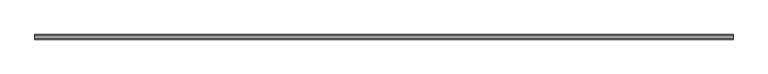
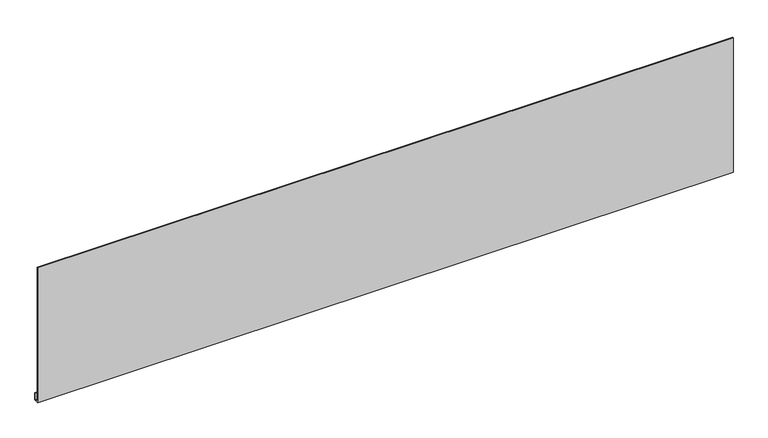
"""IFC4 building model written with IfcOpenShell, lengths in millimetres: proxy geometry, METALFLASHING : METALFLASHING."""

import ifcopenshell
import ifcopenshell.guid

model = None  # the IFC model being written
_history = None  # IfcOwnerHistory: only IFC2X3 demands one
_inside = {}  # id of a spatial element -> (the spatial element, [elements in it])
_under = {}  # id of a project, library or spatial element -> (it, [spatial elements below it])
_declared = {}  # id of a project -> (the project, [libraries it declares])
_typed = {}  # id of a type object -> (the type object, [elements of that type])
_made_of = {}  # id of a material, layer set ... -> (it, [elements and type objects made of it])


def new_model(schema):
    """Start an empty IFC model of exactly this schema.

    Asked for "IFC4X3", IfcOpenShell would pick the latest addendum, in which some entities
    have other attributes; the version numbers below select the first issue.
    IFC2X3 requires an IfcOwnerHistory on every rooted entity: one is made here for all.
    """
    global model, _history
    if schema == "IFC4X3":
        model = ifcopenshell.file(schema_version=(4, 3, 0, 0))
    else:
        model = ifcopenshell.file(schema=schema)
    _inside.clear()
    _under.clear()
    _declared.clear()
    _typed.clear()
    _made_of.clear()
    _history = None
    if model.schema == "IFC2X3":
        org = make("IfcOrganization", Name="unknown")
        user = make(
            "IfcPersonAndOrganization",
            ThePerson=make("IfcPerson", FamilyName="unknown"),
            TheOrganization=org,
        )
        app = make(
            "IfcApplication",
            ApplicationDeveloper=org,
            Version="unknown",
            ApplicationFullName="unknown",
            ApplicationIdentifier="unknown",
        )
        _history = make(
            "IfcOwnerHistory",
            OwningUser=user,
            OwningApplication=app,
            ChangeAction="ADDED",
            CreationDate=0,
        )
    return model


def make(cls, **values):
    """One entity of the class cls with the attributes given. An attribute that is None is left unset."""
    return model.create_entity(
        cls, **{name: value for name, value in values.items() if value is not None}
    )


def rooted(cls, **values):
    """An entity with a GlobalId (a new one), such as an element, a storey or a relation."""
    return make(cls, GlobalId=ifcopenshell.guid.new(), OwnerHistory=_history, **values)


def si_unit(unit_type, name, prefix=None):
    """IfcSIUnit, for example si_unit("LENGTHUNIT", "METRE", prefix="MILLI")."""
    return make("IfcSIUnit", UnitType=unit_type, Prefix=prefix, Name=name)


def assignment(units):
    """IfcUnitAssignment: the units of a project."""
    return None if units is None else make("IfcUnitAssignment", Units=units)


def point(xyz):
    """IfcCartesianPoint."""
    return None if xyz is None else make("IfcCartesianPoint", Coordinates=xyz)


def direction(xyz):
    """IfcDirection."""
    return None if xyz is None else make("IfcDirection", DirectionRatios=xyz)


def frame(location, z_axis=None, x_axis=None):
    """IfcAxis2Placement3D, a coordinate frame: its origin and axes. An axis left out is left unset."""
    return make(
        "IfcAxis2Placement3D",
        Location=point(location),
        Axis=direction(z_axis),
        RefDirection=direction(x_axis),
    )


def origin():
    """The frame at (0, 0, 0) with its axes left unset."""
    return frame((0.0, 0.0, 0.0))


def place(relative_to, where):
    """IfcLocalPlacement: puts the frame where relative to a parent placement (None: the world)."""
    return make(
        "IfcLocalPlacement", PlacementRelTo=relative_to, RelativePlacement=where
    )


def context(
    kind, dimensions, precision=None, world=None, true_north=None, identifier=None
):
    """IfcGeometricRepresentationContext, for example the 3D "Model" context."""
    return make(
        "IfcGeometricRepresentationContext",
        ContextIdentifier=identifier,
        ContextType=kind,
        CoordinateSpaceDimension=dimensions,
        Precision=precision,
        WorldCoordinateSystem=world,
        TrueNorth=true_north,
    )


def project(units=None, contexts=None):
    """IfcProject with its units and contexts."""
    return rooted(
        "IfcProject",
        Name="project",
        RepresentationContexts=contexts,
        UnitsInContext=assignment(units),
    )


def spatial(cls, under=None, at=None, **own):
    """A site, building, storey or space (cls), placed at a placement, below another one or the project."""
    s = rooted(cls, ObjectPlacement=at, **own)
    if under is not None:
        _under.setdefault(under.id(), (under, []))[1].append(s)
    return s


def polyline(points):
    """IfcPolyline through the points."""
    return make("IfcPolyline", Points=[point(p) for p in points])


def outline(outer, holes=None, kind="AREA"):
    """IfcArbitraryClosedProfileDef: a profile drawn as a closed curve; with holes, ...WithVoids."""
    if holes is None:
        return make("IfcArbitraryClosedProfileDef", ProfileType=kind, OuterCurve=outer)
    return make(
        "IfcArbitraryProfileDefWithVoids",
        ProfileType=kind,
        OuterCurve=outer,
        InnerCurves=holes,
    )


def extrude(swept, where, along, depth):
    """IfcExtrudedAreaSolid: the profile swept, set in the frame where, extruded along a direction by depth."""
    return make(
        "IfcExtrudedAreaSolid",
        SweptArea=swept,
        Position=where,
        ExtrudedDirection=direction(along),
        Depth=depth,
    )


def shape(context_of_items, identifier, shape_type, items):
    """IfcShapeRepresentation: the items that make up one representation, for example the "Body"."""
    return make(
        "IfcShapeRepresentation",
        ContextOfItems=context_of_items,
        RepresentationIdentifier=identifier,
        RepresentationType=shape_type,
        Items=items,
    )


def source(mapping_origin, context_of_items, identifier, shape_type, items):
    """IfcRepresentationMap: a shape defined once, which mapped items show again and again."""
    return make(
        "IfcRepresentationMap",
        MappingOrigin=mapping_origin,
        MappedRepresentation=shape(context_of_items, identifier, shape_type, items),
    )


def transform(
    local_origin,
    x_axis=None,
    y_axis=None,
    z_axis=None,
    scale=None,
    scale2=None,
    scale3=None,
    uniform=True,
):
    """IfcCartesianTransformationOperator3D, or its non-uniform kind. x_axis, y_axis, z_axis: its Axis1, 2, 3."""
    if uniform:
        return make(
            "IfcCartesianTransformationOperator3D",
            Axis1=direction(x_axis),
            Axis2=direction(y_axis),
            LocalOrigin=point(local_origin),
            Scale=scale,
            Axis3=direction(z_axis),
        )
    return make(
        "IfcCartesianTransformationOperator3DnonUniform",
        Axis1=direction(x_axis),
        Axis2=direction(y_axis),
        LocalOrigin=point(local_origin),
        Scale=scale,
        Axis3=direction(z_axis),
        Scale2=scale2,
        Scale3=scale3,
    )


def mapped(mapping_source, mapping_target):
    """IfcMappedItem: shows the shape of a source again, moved by a transform."""
    return make(
        "IfcMappedItem", MappingSource=mapping_source, MappingTarget=mapping_target
    )


def made_of(thing, what):
    """Note that an element or type object is made of a material, layer set ...; save() writes the relation."""
    if what is not None:
        _made_of.setdefault(what.id(), (what, []))[1].append(thing)
    return thing


def element(
    cls,
    number,
    at=None,
    inside=None,
    cuts=None,
    type_object=None,
    material=None,
    context=None,
    identifier="Body",
    shape_type=None,
    held_by="IfcProductDefinitionShape",
    body=None,
    shapes=None,
    **own,
):
    """One element of the class cls, such as IfcWall. Its Tag is "e" and its number.

    at: its placement. inside: the storey or other place that contains it. cuts: it is an
    opening in that element (IfcRelVoidsElement). A single representation is given by context,
    identifier, shape_type and body (its items); several are given by shapes. held_by: the class
    of the entity that holds the representations. save() writes the other relations.
    """
    e = rooted(cls, Tag="e%d" % number, ObjectPlacement=at, **own)
    if body is not None:
        shapes = [shape(context, identifier, shape_type, body)]
    if shapes is not None:
        e.Representation = make(held_by, Representations=shapes)
    if inside is not None:
        _inside.setdefault(inside.id(), (inside, []))[1].append(e)
    if cuts is not None:
        rooted(
            "IfcRelVoidsElement", RelatingBuildingElement=cuts, RelatedOpeningElement=e
        )
    if type_object is not None:
        _typed.setdefault(type_object.id(), (type_object, []))[1].append(e)
    return made_of(e, material)


def aggregate(whole, parts):
    """IfcRelAggregates: a whole, such as a stair, and the parts it consists of."""
    return rooted("IfcRelAggregates", RelatingObject=whole, RelatedObjects=parts)


def save(model, path):
    """Write the relations noted so far, then the file.

    IfcRelAggregates (storeys below a building ...), IfcRelContainedInSpatialStructure (elements
    in a storey), IfcRelDefinesByType, IfcRelAssociatesMaterial and IfcRelDeclares: one each for
    every whole, place, type object, material and project.
    """
    for whole, parts in _under.values():
        aggregate(whole, parts)
    for where, things in _inside.values():
        rooted(
            "IfcRelContainedInSpatialStructure",
            RelatedElements=things,
            RelatingStructure=where,
        )
    for kind, things in _typed.values():
        rooted("IfcRelDefinesByType", RelatedObjects=things, RelatingType=kind)
    for what, things in _made_of.values():
        rooted("IfcRelAssociatesMaterial", RelatedObjects=things, RelatingMaterial=what)
    for by, libraries in _declared.values():
        rooted("IfcRelDeclares", RelatingContext=by, RelatedDefinitions=libraries)
    model.write(path)


def generic_models_82097f42(model_context):
    return source(origin(), model_context, "Body", "SweptSolid", [
        extrude(outline(polyline([(-5588.365723, 42324.066406), (-5601.520996, 42324.066406), (-5601.520996, 42733.710938), (-5598.980996, 42733.710938), (-5598.980996, 42326.606406), (-5590.905723, 42326.606406), (-5590.905723, 42345.332031), (-5588.365723, 42345.332031), (-5588.365723, 42324.066406)])), frame((12382.7678845, 0.0, 0.0), z_axis=(1.0, 0.0, 0.0), x_axis=(0.0, 1.0, 0.0)), (0.0, 0.0, 1.0), 2000.25),
    ])


if __name__ == "__main__":
    model = new_model("IFC4")
    model_context = context("Model", 3, world=origin())
    ifc_project = project(units=[si_unit("LENGTHUNIT", "METRE", prefix="MILLI")], contexts=[model_context])
    site = spatial("IfcSite", under=ifc_project)
    building = spatial("IfcBuilding", under=site)
    placement = place(None, origin())
    generic_models_shape = generic_models_82097f42(model_context)
    element("IfcBuildingElementProxy", 1, Name="METALFLASHING : METALFLASHING", ObjectType="METALFLASHING : METALFLASHING", at=placement, inside=building, context=model_context, shape_type="MappedRepresentation", body=[
        mapped(generic_models_shape, transform((0.0, 0.0, 0.0), x_axis=(1.0, 0.0, 0.0), y_axis=(0.0, 1.0, 0.0), z_axis=(0.0, 0.0, 1.0))),
    ])
    save(model, "model.ifc")

# Revit data of these elements
# Type "METALFLASHING : METALFLASHING"
#   NameOverride = "METALFLASHING"
# Element 1 (IfcBuildingElementProxy, "METALFLASHING : METALFLASHING")
#   Materials on its faces: "BRAKE METAL EAVE TRIM TO MATCH STANDING SEAM COLOR"
# Materials
#   "BRAKE METAL EAVE TRIM TO MATCH STANDING SEAM COLOR": class "Unassigned", colour RGB 128 128 128, transparency 0, Cost = 0
